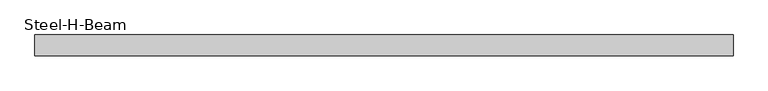
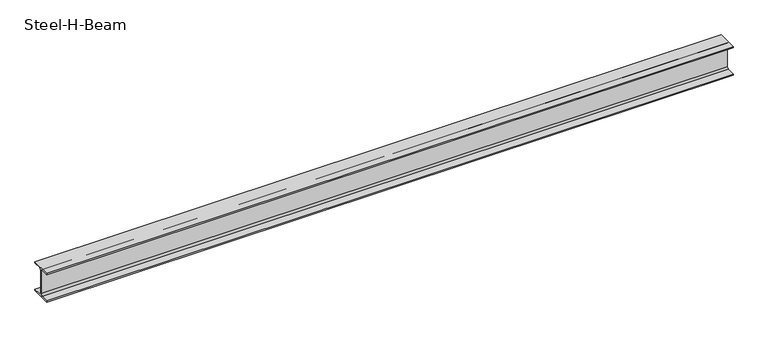
"""IFC4 building model written with IfcOpenShell, lengths in millimetres: beam geometry, Steel-H-Beam : BM121_H-294×200x8x12."""

from ifc_helpers import new_model, si_unit, point, frame, frame_2d, origin, place, context, project, spatial, polyline, circle_curve, trimmed, segment, composite_curve, outline, extrude, source, transform, mapped, element, save


def steel_h_beam_3e669b2c(model_context):
    return source(origin(), model_context, "Body", "SweptSolid", [
        extrude(outline(composite_curve([segment(polyline([(100.0, -135.0), (100.0, -147.0), (-100.0, -147.0), (-100.0, -135.0), (-22.0, -135.0)]), True, "CONTINUOUS"), segment(trimmed(circle_curve(frame_2d((-22.0, -117.0)), 18.0), [point((-22.0, -135.0))], [point((-4.0, -117.0))], True, "CARTESIAN"), True, "CONTINUOUS"), segment(polyline([(-4.0, -117.0), (-4.0, 117.0)]), True, "CONTINUOUS"), segment(trimmed(circle_curve(frame_2d((-22.0, 117.0)), 18.0), [point((-4.0, 117.0))], [point((-22.0, 135.0))], True, "CARTESIAN"), True, "CONTINUOUS"), segment(polyline([(-22.0, 135.0), (-100.0, 135.0), (-100.0, 147.0), (100.0, 147.0), (100.0, 135.0), (22.0, 135.0)]), True, "CONTINUOUS"), segment(trimmed(circle_curve(frame_2d((22.0, 117.0)), 18.0), [point((22.0, 135.0))], [point((4.0, 117.0))], True, "CARTESIAN"), True, "CONTINUOUS"), segment(polyline([(4.0, 117.0), (4.0, -117.0)]), True, "CONTINUOUS"), segment(trimmed(circle_curve(frame_2d((22.0, -117.0)), 18.0), [point((4.0, -117.0))], [point((22.0, -135.0))], True, "CARTESIAN"), True, "CONTINUOUS"), segment(polyline([(22.0, -135.0), (100.0, -135.0)]), True, "CONTINUOUS")], self_intersect=False)), frame((-3500.0, 0.0, 0.0), z_axis=(1.0, 0.0, 0.0), x_axis=(0.0, 1.0, 0.0)), (0.0, 0.0, 1.0), 6687.2337007),
    ])


if __name__ == "__main__":
    model = new_model("IFC4")
    model_context = context("Model", 3, world=origin())
    ifc_project = project(units=[si_unit("LENGTHUNIT", "METRE", prefix="MILLI")], contexts=[model_context])
    site = spatial("IfcSite", under=ifc_project)
    building = spatial("IfcBuilding", under=site)
    placement = place(None, origin())
    steel_h_beam_shape = steel_h_beam_3e669b2c(model_context)
    element("IfcBeam", 1, ObjectType="Steel-H-Beam : BM121_H-294×200x8x12", at=placement, inside=building, context=model_context, shape_type="MappedRepresentation", body=[
        mapped(steel_h_beam_shape, transform((0.0, 0.0, 0.0), x_axis=(1.0, 0.0, 0.0), y_axis=(0.0, 1.0, 0.0), z_axis=(0.0, 0.0, 1.0))),
    ])
    save(model, "model.ifc")

# Revit data of these elements
# Type "Steel-H-Beam : BM121_H-294×200x8x12"
#   Surface Area = 1.3411 m²/m
#   Section Area = 72.3812 cm²
#   Mass per Unit Length = 56.8193 kg/m
#   Length [instance default] = 3000 mm
#   B = 200 mm
#   H = 294 mm
#   r = 18 mm
#   tw = 8 mm
#   tf = 12 mm
#   hec_material4 [instance default] = none
#   hec_material3 [instance default] = none
#   hec_material2 [instance default] = none
#   hec_material1 [instance default] = none
#   Structural Material [instance default] = Steel, 45-345
#   Assembly Code = ""
# Element 1 (IfcBeam, "Steel-H-Beam : BM121_H-294×200x8x12")
#   hec_material3 = F01AC000-00002_Building/Shelter Fire Proofing Work_Intumescent Coating Type_1 hr. rating (UL 1709))
#   hec_material2 = S01AA010-00002_Main Steel Structure Fabrication Work_Shelter/Building_Steel Painting/Coating_for Fireproofed Steel Surface, Surface Preparation & Primer Coat
#   hec_material1 = S03AA028-00001_Main Steel Structure Erection Work_Shelter/Building_Medium Steel
#   Structural Material = S01AA002-00001_Main Steel Structure Fabrication Work_Shelter/Building_Medium Steel - Standard
#   Materials on its faces: "S01AA002-00001_Main Steel Structure Fabrication Work_Shelter/Building_Medium Steel - Standard"
# Materials
#   "Steel, 45-345": class "Metal", colour RGB 189 187 185, transparency 0, Description = "Steel 345 MPa", Cost = 0
#   "S01AA002-00001_Main Steel Structure Fabrication Work_Shelter/Building_Medium Steel - Standard": class "Metal", colour RGB 120 120 120, transparency 0, Comments = "(90KG/M>Weight≥30KG/M)", Description = "Structural steel 50ksi", W00) Work Master Code = "S01AA002-0001", W01) Work Master_Lv1 = "Main Steel Structure Fabrication Work", W02) Work Master_Lv2 = "Shelter/Building", W03) Work Master_Spec.1 = "Medium Steel - Standard (90KG/M>Weight≥30KG/M)", Cost = 0
#   "F01AC000-00002_Building/Shelter Fire Proofing Work_Intumescent Coating Type_1 hr. rating (UL 1709))": class "Metal", colour RGB 255 128 128, transparency 0, Description = "Paint finished steel", W00) Work Master Code = "F01AC000-00002", W01) Work Master_Lv1 = "Building/Shelter Fire Proofing Work", W02) Work Master_Lv2 = "Intumescent Coating Type", W03) Work Master_Spec.1 = "1 hr. rating (UL 1709)", Cost = 0
#   "S01AA010-00002_Main Steel Structure Fabrication Work_Shelter/Building_Steel Painting/Coating_for Fireproofed Steel Surface, Surface Preparation & Primer Coat": class "Metal", colour RGB 120 120 120, transparency 0, Description = "Paint finished steel", W00) Work Master Code = "SS01AA010-00002", W01) Work Master_Lv1 = "Main Steel Structure Fabrication Work", W02) Work Master_Lv2 = "Shelter/Building", W03) Work Master_Spec.1 = "Steel Painting/Coating", W04) Work Master_Spec.2 = "for Fireproofed Steel Surface, Surface Preparation & Primer Coat", Cost = 0
#   "S03AA028-00001_Main Steel Structure Erection Work_Shelter/Building_Medium Steel": class "Metal", colour RGB 120 120 120, transparency 0, Comments = "(90KG/M>Weight≥30KG/M)", Description = "Structural steel 50ksi", W00) Work Master Code = "S03AA028-0001", W01) Work Master_Lv1 = "Main Steel Structure Erection Work", W02) Work Master_Lv2 = "Shelter/Building", W03) Work Master_Spec.1 = "Medium Steel (90KG/M>Weight≥30KG/M)", Cost = 0
